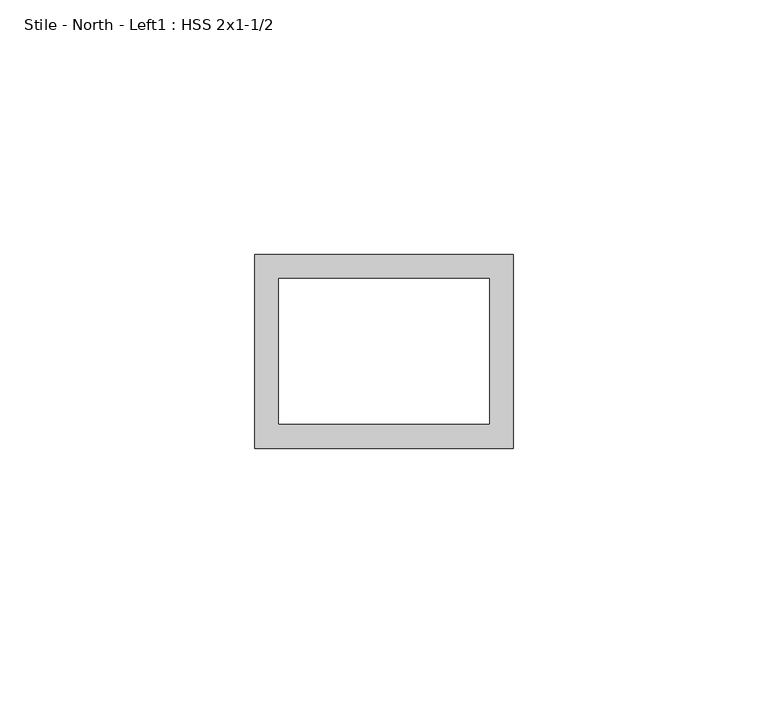
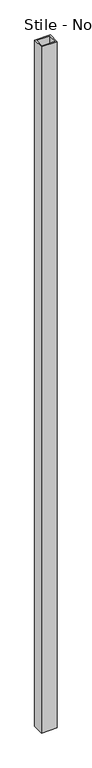
"""IFC4 building model written with IfcOpenShell, lengths in millimetres: proxy geometry, Stile - North - Left1 : HSS 2x1-1/2."""

from ifc_helpers import new_model, si_unit, frame, origin, place, context, project, spatial, polyline, outline, extrude, source, transform, mapped, element, save


def stile_north_left1_hss_2x1_1_2_870a2a95(model_context):
    return source(origin(), model_context, "Body", "SweptSolid", [
        extrude(outline(polyline([(587365.8934739, -534109.3663841), (587416.6934739, -534109.3663841), (587416.6934739, -534147.4663841), (587365.8934739, -534147.4663841), (587365.8934739, -534109.3663841)]), holes=[polyline([(587370.6559739, -534114.1288841), (587370.6559739, -534142.7038841), (587411.9309739, -534142.7038841), (587411.9309739, -534114.1288841), (587370.6559739, -534114.1288841)])]), frame((0.0, 0.0, 50.8), z_axis=(0.0, 0.0, 1.0), x_axis=(1.0, 0.0, 0.0)), (0.0, 0.0, 1.0), 2349.5),
    ])


if __name__ == "__main__":
    model = new_model("IFC4")
    model_context = context("Model", 3, world=origin())
    ifc_project = project(units=[si_unit("LENGTHUNIT", "METRE", prefix="MILLI")], contexts=[model_context])
    site = spatial("IfcSite", under=ifc_project)
    building = spatial("IfcBuilding", under=site)
    placement = place(None, origin())
    stile_north_left1_hss_2x1_1_2_shape = stile_north_left1_hss_2x1_1_2_870a2a95(model_context)
    element("IfcBuildingElementProxy", 1, Name="Stile - North - Left1 : HSS 2x1-1/2", ObjectType="Stile - North - Left1 : HSS 2x1-1/2", at=placement, inside=building, context=model_context, shape_type="MappedRepresentation", body=[
        mapped(stile_north_left1_hss_2x1_1_2_shape, transform((0.0, 0.0, 0.0), x_axis=(1.0, 0.0, 0.0), y_axis=(0.0, 1.0, 0.0), z_axis=(0.0, 0.0, 1.0))),
    ])
    save(model, "model.ifc")

# Revit data of these elements
# Element 1 (IfcBuildingElementProxy, "Stile - North - Left1 : HSS 2x1-1/2")
#   Materials on its faces: "1-1/2\"X2\" GALV. STL HSS TUBING"
# Materials
#   "1-1/2\"X2\" GALV. STL HSS TUBING": class "Generic", colour RGB 211 211 207, transparency 0, Cost = 0
